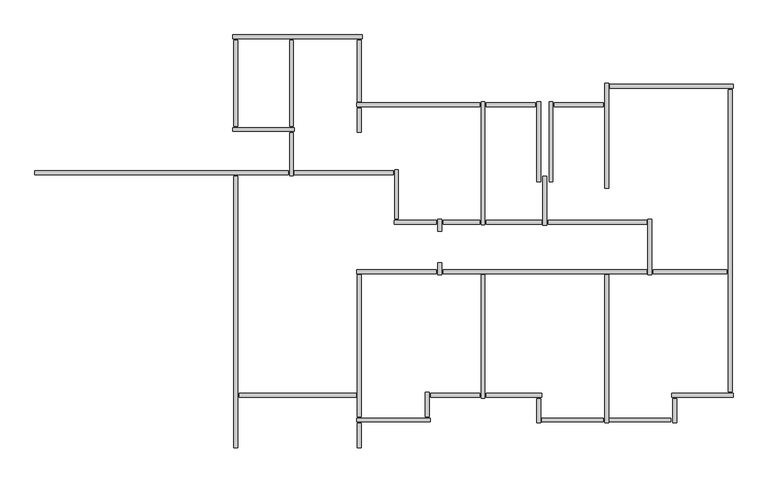
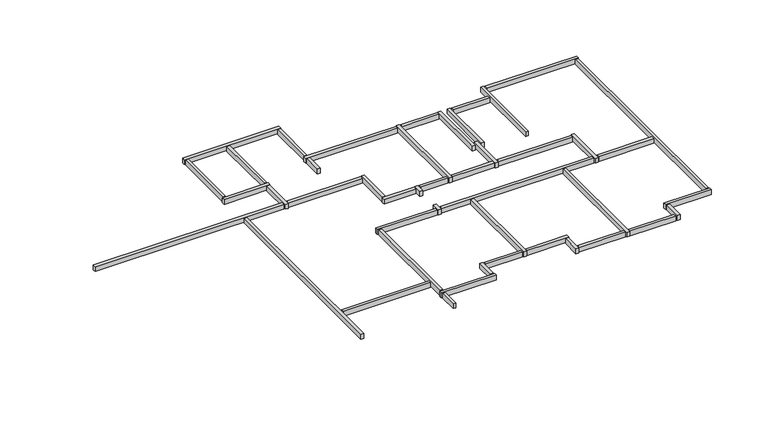
"""IFC4 building model written with IfcOpenShell, lengths in millimetres: beam geometry, Graute viga de respaldo : Graute viga de respaldo."""

from ifc_helpers import new_model, si_unit, frame, origin, place, context, project, spatial, polyline, outline, extrude, source, transform, mapped, element, save


def beam_bbf57b8f(model_context):
    return source(origin(), model_context, "Body", "SweptSolid", [
        extrude(outline(polyline([(-54994.9587292, 57408.4278788), (-54994.9587292, 57502.4278788), (-53804.9587292, 57502.4278788), (-53804.9587292, 57408.4278788), (-54994.9587292, 57408.4278788)])), frame((0.0, 0.0, 2632.9999999), z_axis=(0.0, 0.0, 1.0), x_axis=(1.0, 0.0, 0.0)), (0.0, 0.0, 1.0), 167.0),
        extrude(outline(polyline([(-56644.9587292, 57408.4278788), (-56644.9587292, 57502.4278788), (-55454.9587292, 57502.4278788), (-55454.9587292, 57408.4278788), (-56644.9587292, 57408.4278788)])), frame((0.0, 0.0, 2632.9999999), z_axis=(0.0, 0.0, 1.0), x_axis=(1.0, 0.0, 0.0)), (0.0, 0.0, 1.0), 167.0),
        extrude(outline(polyline([(-52594.9587292, 53358.4278788), (-52594.9587292, 53452.4278788), (-50804.9587292, 53452.4278788), (-50804.9587292, 53358.4278788), (-52594.9587292, 53358.4278788)])), frame((0.0, 0.0, 2632.9999999), z_axis=(0.0, 0.0, 1.0), x_axis=(1.0, 0.0, 0.0)), (0.0, 0.0, 1.0), 167.0),
        extrude(outline(polyline([(-57994.9587292, 50358.4278788), (-57994.9587292, 50452.4278788), (-56804.9587292, 50452.4278788), (-56804.9587292, 50358.4278788), (-57994.9587292, 50358.4278788)])), frame((0.0, 0.0, 2632.9999999), z_axis=(0.0, 0.0, 1.0), x_axis=(1.0, 0.0, 0.0)), (0.0, 0.0, 1.0), 167.0),
        extrude(outline(polyline([(-58121.9587292, 50475.4278788), (-58027.9587292, 50475.4278788), (-58027.9587292, 49885.4278788), (-58121.9587292, 49885.4278788), (-58121.9587292, 50475.4278788)])), frame((0.0, 0.0, 2632.9999999), z_axis=(0.0, 0.0, 1.0), x_axis=(1.0, 0.0, 0.0)), (0.0, 0.0, 1.0), 167.0),
        extrude(outline(polyline([(-59794.9587292, 49758.4278788), (-59794.9587292, 49852.4278788), (-58004.9587292, 49852.4278788), (-58004.9587292, 49758.4278788), (-59794.9587292, 49758.4278788)])), frame((0.0, 0.0, 2632.9999999), z_axis=(0.0, 0.0, 1.0), x_axis=(1.0, 0.0, 0.0)), (0.0, 0.0, 1.0), 167.0),
        extrude(outline(polyline([(-57727.9587292, 53335.4278788), (-57821.9587292, 53335.4278788), (-57821.9587292, 53625.4278788), (-57727.9587292, 53625.4278788), (-57727.9587292, 53335.4278788)])), frame((0.0, 0.0, 2632.9999999), z_axis=(0.0, 0.0, 1.0), x_axis=(1.0, 0.0, 0.0)), (0.0, 0.0, 1.0), 167.0),
        extrude(outline(polyline([(-55144.9587292, 54558.4278788), (-55144.9587292, 54652.4278788), (-52754.9587292, 54652.4278788), (-52754.9587292, 54558.4278788), (-55144.9587292, 54558.4278788)])), frame((0.0, 0.0, 2632.9999999), z_axis=(0.0, 0.0, 1.0), x_axis=(1.0, 0.0, 0.0)), (0.0, 0.0, 1.0), 167.0),
        extrude(outline(polyline([(-56644.9587292, 54558.4278788), (-56644.9587292, 54652.4278788), (-55304.9587292, 54652.4278788), (-55304.9587292, 54558.4278788), (-56644.9587292, 54558.4278788)])), frame((0.0, 0.0, 2632.9999999), z_axis=(0.0, 0.0, 1.0), x_axis=(1.0, 0.0, 0.0)), (0.0, 0.0, 1.0), 167.0),
        extrude(outline(polyline([(-57694.9587292, 54558.4278788), (-57694.9587292, 54652.4278788), (-56804.9587292, 54652.4278788), (-56804.9587292, 54558.4278788), (-57694.9587292, 54558.4278788)])), frame((0.0, 0.0, 2632.9999999), z_axis=(0.0, 0.0, 1.0), x_axis=(1.0, 0.0, 0.0)), (0.0, 0.0, 1.0), 167.0),
        extrude(outline(polyline([(-57727.9587292, 54385.4278788), (-57821.9587292, 54385.4278788), (-57821.9587292, 54675.4278788), (-57727.9587292, 54675.4278788), (-57727.9587292, 54385.4278788)])), frame((0.0, 0.0, 2632.9999999), z_axis=(0.0, 0.0, 1.0), x_axis=(1.0, 0.0, 0.0)), (0.0, 0.0, 1.0), 167.0),
        extrude(outline(polyline([(-58884.9587292, 54558.4278788), (-58884.9587292, 54652.4278788), (-57854.9587292, 54652.4278788), (-57854.9587292, 54558.4278788), (-58884.9587292, 54558.4278788)])), frame((0.0, 0.0, 2632.9999999), z_axis=(0.0, 0.0, 1.0), x_axis=(1.0, 0.0, 0.0)), (0.0, 0.0, 1.0), 167.0),
        extrude(outline(polyline([(-58871.9587292, 55875.4278788), (-58777.9587292, 55875.4278788), (-58777.9587292, 54685.4278788), (-58871.9587292, 54685.4278788), (-58871.9587292, 55875.4278788)])), frame((0.0, 0.0, 2632.9999999), z_axis=(0.0, 0.0, 1.0), x_axis=(1.0, 0.0, 0.0)), (0.0, 0.0, 1.0), 167.0),
        extrude(outline(polyline([(-61304.9587292, 55758.4278788), (-61304.9587292, 55852.4278788), (-58904.9587292, 55852.4278788), (-58904.9587292, 55758.4278788), (-61304.9587292, 55758.4278788)])), frame((0.0, 0.0, 2632.9999999), z_axis=(0.0, 0.0, 1.0), x_axis=(1.0, 0.0, 0.0)), (0.0, 0.0, 1.0), 167.0),
        extrude(outline(polyline([(-56677.9587292, 54540.4278788), (-56771.9587292, 54540.4278788), (-56771.9587292, 57525.4278788), (-56677.9587292, 57525.4278788), (-56677.9587292, 54540.4278788)])), frame((0.0, 0.0, 2632.9999999), z_axis=(0.0, 0.0, 1.0), x_axis=(1.0, 0.0, 0.0)), (0.0, 0.0, 1.0), 167.0),
        extrude(outline(polyline([(-59794.9587292, 57408.4278788), (-59794.9587292, 57502.4278788), (-56804.9587292, 57502.4278788), (-56804.9587292, 57408.4278788), (-59794.9587292, 57408.4278788)])), frame((0.0, 0.0, 2632.9999999), z_axis=(0.0, 0.0, 1.0), x_axis=(1.0, 0.0, 0.0)), (0.0, 0.0, 1.0), 167.0),
        extrude(outline(polyline([(-59677.9587292, 56785.4278788), (-59771.9587292, 56785.4278788), (-59771.9587292, 57375.4278788), (-59677.9587292, 57375.4278788), (-59677.9587292, 56785.4278788)])), frame((0.0, 0.0, 2632.9999999), z_axis=(0.0, 0.0, 1.0), x_axis=(1.0, 0.0, 0.0)), (0.0, 0.0, 1.0), 167.0),
        extrude(outline(polyline([(-59771.9587292, 59025.4278788), (-59677.9587292, 59025.4278788), (-59677.9587292, 57535.4278788), (-59771.9587292, 57535.4278788), (-59771.9587292, 59025.4278788)])), frame((0.0, 0.0, 2632.9999999), z_axis=(0.0, 0.0, 1.0), x_axis=(1.0, 0.0, 0.0)), (0.0, 0.0, 1.0), 167.0),
        extrude(outline(polyline([(-62771.9587292, 59025.4278788), (-62677.9587292, 59025.4278788), (-62677.9587292, 56935.4278788), (-62771.9587292, 56935.4278788), (-62771.9587292, 59025.4278788)])), frame((0.0, 0.0, 2632.9999999), z_axis=(0.0, 0.0, 1.0), x_axis=(1.0, 0.0, 0.0)), (0.0, 0.0, 1.0), 167.0),
        extrude(outline(polyline([(-61421.9587292, 59025.4278788), (-61327.9587292, 59025.4278788), (-61327.9587292, 56935.4278788), (-61421.9587292, 56935.4278788), (-61421.9587292, 59025.4278788)])), frame((0.0, 0.0, 2632.9999999), z_axis=(0.0, 0.0, 1.0), x_axis=(1.0, 0.0, 0.0)), (0.0, 0.0, 1.0), 167.0),
        extrude(outline(polyline([(-61327.9587292, 55735.4278788), (-61421.9587292, 55735.4278788), (-61421.9587292, 56775.4278788), (-61327.9587292, 56775.4278788), (-61327.9587292, 55735.4278788)])), frame((0.0, 0.0, 2632.9999999), z_axis=(0.0, 0.0, 1.0), x_axis=(1.0, 0.0, 0.0)), (0.0, 0.0, 1.0), 167.0),
        extrude(outline(polyline([(-62644.9587292, 50358.4278788), (-62644.9587292, 50452.4278788), (-59804.9587292, 50452.4278788), (-59804.9587292, 50358.4278788), (-62644.9587292, 50358.4278788)])), frame((0.0, 0.0, 2632.9999999), z_axis=(0.0, 0.0, 1.0), x_axis=(1.0, 0.0, 0.0)), (0.0, 0.0, 1.0), 167.0),
        extrude(outline(polyline([(-59771.9587292, 53325.4278788), (-59677.9587292, 53325.4278788), (-59677.9587292, 49885.4278788), (-59771.9587292, 49885.4278788), (-59771.9587292, 53325.4278788)])), frame((0.0, 0.0, 2632.9999999), z_axis=(0.0, 0.0, 1.0), x_axis=(1.0, 0.0, 0.0)), (0.0, 0.0, 1.0), 167.0),
        extrude(outline(polyline([(-59794.9587292, 53358.4278788), (-59794.9587292, 53452.4278788), (-57854.9587292, 53452.4278788), (-57854.9587292, 53358.4278788), (-59794.9587292, 53358.4278788)])), frame((0.0, 0.0, 2632.9999999), z_axis=(0.0, 0.0, 1.0), x_axis=(1.0, 0.0, 0.0)), (0.0, 0.0, 1.0), 167.0),
        extrude(outline(polyline([(-57694.9587292, 53358.4278788), (-57694.9587292, 53452.4278788), (-52754.9587292, 53452.4278788), (-52754.9587292, 53358.4278788), (-57694.9587292, 53358.4278788)])), frame((0.0, 0.0, 2632.9999999), z_axis=(0.0, 0.0, 1.0), x_axis=(1.0, 0.0, 0.0)), (0.0, 0.0, 1.0), 167.0),
        extrude(outline(polyline([(-56677.9587292, 50335.4278788), (-56771.9587292, 50335.4278788), (-56771.9587292, 53325.4278788), (-56677.9587292, 53325.4278788), (-56677.9587292, 50335.4278788)])), frame((0.0, 0.0, 2632.9999999), z_axis=(0.0, 0.0, 1.0), x_axis=(1.0, 0.0, 0.0)), (0.0, 0.0, 1.0), 167.0),
        extrude(outline(polyline([(-55304.9587292, 50452.4278788), (-55304.9587292, 50358.4278788), (-56644.9587292, 50358.4278788), (-56644.9587292, 50452.4278788), (-55304.9587292, 50452.4278788)])), frame((0.0, 0.0, 2632.9999999), z_axis=(0.0, 0.0, 1.0), x_axis=(1.0, 0.0, 0.0)), (0.0, 0.0, 1.0), 167.0),
        extrude(outline(polyline([(-55327.9587292, 49735.4278788), (-55421.9587292, 49735.4278788), (-55421.9587292, 50325.4278788), (-55327.9587292, 50325.4278788), (-55327.9587292, 49735.4278788)])), frame((0.0, 0.0, 2632.9999999), z_axis=(0.0, 0.0, 1.0), x_axis=(1.0, 0.0, 0.0)), (0.0, 0.0, 1.0), 167.0),
        extrude(outline(polyline([(-55294.9587292, 49758.4278788), (-55294.9587292, 49852.4278788), (-53804.9587292, 49852.4278788), (-53804.9587292, 49758.4278788), (-55294.9587292, 49758.4278788)])), frame((0.0, 0.0, 2632.9999999), z_axis=(0.0, 0.0, 1.0), x_axis=(1.0, 0.0, 0.0)), (0.0, 0.0, 1.0), 167.0),
        extrude(outline(polyline([(-52165.9809043, 49853.4278788), (-52165.9809043, 49758.4278788), (-53654.9587292, 49758.4278788), (-53654.9587292, 49853.4278788), (-52165.9809043, 49853.4278788)])), frame((0.0, 0.0, 2617.1856208), z_axis=(0.0, 0.0, 1.0), x_axis=(1.0, 0.0, 0.0)), (0.0, 0.0, 1.0), 165.0),
        extrude(outline(polyline([(-50771.9587292, 57825.4278788), (-50677.9587292, 57825.4278788), (-50677.9587292, 50485.4278788), (-50771.9587292, 50485.4278788), (-50771.9587292, 57825.4278788)])), frame((0.0, 0.0, 2632.9999999), z_axis=(0.0, 0.0, 1.0), x_axis=(1.0, 0.0, 0.0)), (0.0, 0.0, 1.0), 167.0),
        extrude(outline(polyline([(-52721.9587292, 54675.4278788), (-52627.9587292, 54675.4278788), (-52627.9587292, 53330.0746661), (-52721.9587292, 53330.0746661), (-52721.9587292, 54675.4278788)])), frame((0.0, 0.0, 2632.9999999), z_axis=(0.0, 0.0, 1.0), x_axis=(1.0, 0.0, 0.0)), (0.0, 0.0, 1.0), 167.0),
        extrude(outline(polyline([(-55271.9587292, 55725.4278788), (-55177.9587292, 55725.4278788), (-55177.9587292, 54535.4278788), (-55271.9587292, 54535.4278788), (-55271.9587292, 55725.4278788)])), frame((0.0, 0.0, 2632.9999999), z_axis=(0.0, 0.0, 1.0), x_axis=(1.0, 0.0, 0.0)), (0.0, 0.0, 1.0), 167.0),
        extrude(outline(polyline([(-55121.9587292, 57525.4278788), (-55027.9587292, 57525.4278788), (-55027.9587292, 55585.4278788), (-55121.9587292, 55585.4278788), (-55121.9587292, 57525.4278788)])), frame((0.0, 0.0, 2632.9999999), z_axis=(0.0, 0.0, 1.0), x_axis=(1.0, 0.0, 0.0)), (0.0, 0.0, 1.0), 167.0),
        extrude(outline(polyline([(-55421.9587292, 57525.4278788), (-55327.9587292, 57525.4278788), (-55327.9587292, 55585.4278788), (-55421.9587292, 55585.4278788), (-55421.9587292, 57525.4278788)])), frame((0.0, 0.0, 2632.9999999), z_axis=(0.0, 0.0, 1.0), x_axis=(1.0, 0.0, 0.0)), (0.0, 0.0, 1.0), 167.0),
        extrude(outline(polyline([(-53771.9587292, 57975.4278788), (-53677.9587292, 57975.4278788), (-53677.9587292, 55435.4278788), (-53771.9587292, 55435.4278788), (-53771.9587292, 57975.4278788)])), frame((0.0, 0.0, 2632.9999999), z_axis=(0.0, 0.0, 1.0), x_axis=(1.0, 0.0, 0.0)), (0.0, 0.0, 1.0), 167.0),
        extrude(outline(polyline([(-50654.9587292, 57952.4278788), (-50654.9587292, 57858.4278788), (-53644.9587292, 57858.4278788), (-53644.9587292, 57952.4278788), (-50654.9587292, 57952.4278788)])), frame((0.0, 0.0, 2632.9999999), z_axis=(0.0, 0.0, 1.0), x_axis=(1.0, 0.0, 0.0)), (0.0, 0.0, 1.0), 167.0),
        extrude(outline(polyline([(-52027.9587292, 49735.4278788), (-52121.9587292, 49735.4278788), (-52121.9587292, 50325.4278788), (-52027.9587292, 50325.4278788), (-52027.9587292, 49735.4278788)])), frame((0.0, 0.0, 2632.9999999), z_axis=(0.0, 0.0, 1.0), x_axis=(1.0, 0.0, 0.0)), (0.0, 0.0, 1.0), 167.0),
        extrude(outline(polyline([(-52144.9587292, 50358.4278788), (-52144.9587292, 50452.4278788), (-50654.9587292, 50452.4278788), (-50654.9587292, 50358.4278788), (-52144.9587292, 50358.4278788)])), frame((0.0, 0.0, 2632.9999999), z_axis=(0.0, 0.0, 1.0), x_axis=(1.0, 0.0, 0.0)), (0.0, 0.0, 1.0), 167.0),
        extrude(outline(polyline([(-53677.9587292, 49735.4278788), (-53771.9587292, 49735.4278788), (-53771.9587292, 53325.4278788), (-53677.9587292, 53325.4278788), (-53677.9587292, 49735.4278788)])), frame((0.0, 0.0, 2632.9999999), z_axis=(0.0, 0.0, 1.0), x_axis=(1.0, 0.0, 0.0)), (0.0, 0.0, 1.0), 167.0),
        extrude(outline(polyline([(-59677.9587292, 49135.4278788), (-59771.9587292, 49135.4278788), (-59771.9587292, 49725.4278788), (-59677.9587292, 49725.4278788), (-59677.9587292, 49135.4278788)])), frame((0.0, 0.0, 2632.9999999), z_axis=(0.0, 0.0, 1.0), x_axis=(1.0, 0.0, 0.0)), (0.0, 0.0, 1.0), 167.0),
        extrude(outline(polyline([(-62794.9587292, 56808.4278788), (-62794.9587292, 56902.4278788), (-61304.9587292, 56902.4278788), (-61304.9587292, 56808.4278788), (-62794.9587292, 56808.4278788)])), frame((0.0, 0.0, 2632.9999999), z_axis=(0.0, 0.0, 1.0), x_axis=(1.0, 0.0, 0.0)), (0.0, 0.0, 1.0), 167.0),
        extrude(outline(polyline([(-62794.9587292, 59058.4278788), (-62794.9587292, 59152.4278788), (-59654.9587292, 59152.4278788), (-59654.9587292, 59058.4278788), (-62794.9587292, 59058.4278788)])), frame((0.0, 0.0, 2632.9999999), z_axis=(0.0, 0.0, 1.0), x_axis=(1.0, 0.0, 0.0)), (0.0, 0.0, 1.0), 167.0),
        extrude(outline(polyline([(-67601.7587292, 55758.4278788), (-67601.7587292, 55852.4278788), (-61454.9587292, 55852.4278788), (-61454.9587292, 55758.4278788), (-67601.7587292, 55758.4278788)])), frame((0.0, 0.0, 2632.9999999), z_axis=(0.0, 0.0, 1.0), x_axis=(1.0, 0.0, 0.0)), (0.0, 0.0, 1.0), 167.0),
        extrude(outline(polyline([(-62677.9587292, 49132.8979841), (-62771.9587292, 49132.8979841), (-62771.9587292, 55725.4278788), (-62677.9587292, 55725.4278788), (-62677.9587292, 49132.8979841)])), frame((0.0, 0.0, 2632.9999999), z_axis=(0.0, 0.0, 1.0), x_axis=(1.0, 0.0, 0.0)), (0.0, 0.0, 1.0), 167.0),
    ])


if __name__ == "__main__":
    model = new_model("IFC4")
    model_context = context("Model", 3, world=origin())
    ifc_project = project(units=[si_unit("LENGTHUNIT", "METRE", prefix="MILLI")], contexts=[model_context])
    site = spatial("IfcSite", under=ifc_project)
    building = spatial("IfcBuilding", under=site)
    placement = place(None, origin())
    beam_shape = beam_bbf57b8f(model_context)
    element("IfcBeam", 1, ObjectType="Graute viga de respaldo : Graute viga de respaldo", at=placement, inside=building, context=model_context, shape_type="MappedRepresentation", body=[
        mapped(beam_shape, transform((0.0, 0.0, 0.0), x_axis=(1.0, 0.0, 0.0), y_axis=(0.0, 1.0, 0.0), z_axis=(0.0, 0.0, 1.0))),
    ])
    save(model, "model.ifc")

# Revit data of these elements
# Element 1 (IfcBeam, "Graute viga de respaldo : Graute viga de respaldo")
#   Materials on its faces: "Concreto, Faixa de areia/cimento"
# Materials
#   "Concreto, Faixa de areia/cimento": class "Concreto", colour RGB 127 127 127, transparency 0, Description = "Revestimento de laje de concreto", Cost = 0
